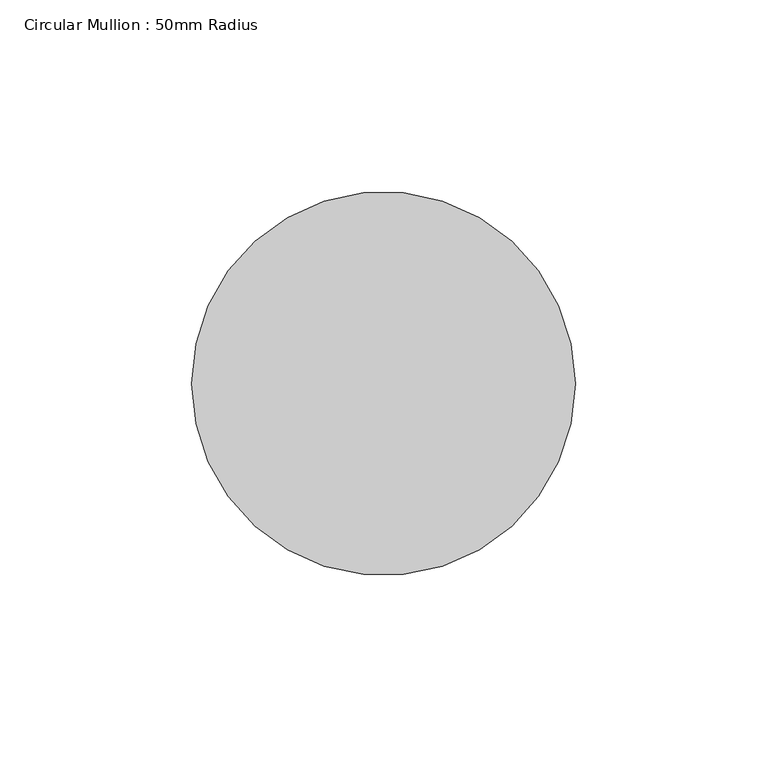
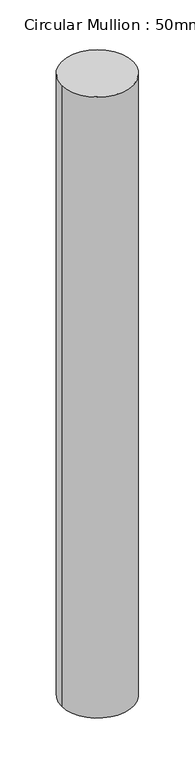
"""IFC4 building model written with IfcOpenShell, lengths in millimetres: member geometry, Circular Mullion : 50mm Radius."""

from ifc_helpers import new_model, si_unit, point, frame, origin, origin_2d, place, context, project, spatial, circle_curve, trimmed, segment, composite_curve, outline, extrude, source, transform, mapped, element, save


def circular_mullion_50mm_radius_25e7e1fa(model_context):
    return source(origin(), model_context, "Body", "SweptSolid", [
        extrude(outline(composite_curve([segment(trimmed(circle_curve(origin_2d(), 50.0), [point((50.0, 0.0))], [point((-50.0, 0.0))], False, "CARTESIAN"), True, "CONTINUOUS"), segment(trimmed(circle_curve(origin_2d(), 50.0), [point((-50.0, 0.0))], [point((50.0, 0.0))], False, "CARTESIAN"), True, "CONTINUOUS")], self_intersect=False)), frame((0.0, 0.0, -920.8984587), z_axis=(0.0, 0.0, 1.0), x_axis=(1.0, 0.0, 0.0)), (0.0, 0.0, 1.0), 920.8984587),
    ])


if __name__ == "__main__":
    model = new_model("IFC4")
    model_context = context("Model", 3, world=origin())
    ifc_project = project(units=[si_unit("LENGTHUNIT", "METRE", prefix="MILLI")], contexts=[model_context])
    site = spatial("IfcSite", under=ifc_project)
    building = spatial("IfcBuilding", under=site)
    placement = place(None, origin())
    circular_mullion_50mm_radius_shape = circular_mullion_50mm_radius_25e7e1fa(model_context)
    element("IfcMember", 1, ObjectType="Circular Mullion : 50mm Radius", at=placement, inside=building, context=model_context, shape_type="MappedRepresentation", body=[
        mapped(circular_mullion_50mm_radius_shape, transform((0.0, 0.0, 0.0), x_axis=(1.0, 0.0, 0.0), y_axis=(0.0, 1.0, 0.0), z_axis=(0.0, 0.0, 1.0))),
    ])
    save(model, "model.ifc")

# Revit data of these elements
# Type "Circular Mullion : 50mm Radius"
#   built-in parameter 1007350 = 0.164042 (stored number, unit not read)
# Element 1 (IfcMember, "Circular Mullion : 50mm Radius")
#   Materials on its faces: "Aluminium"
# Materials
#   "Aluminium": class "Metal", colour RGB 247 247 247, transparency 0, Description = "Aluminium 6061", Cost = 0
